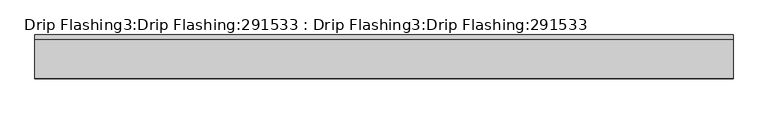
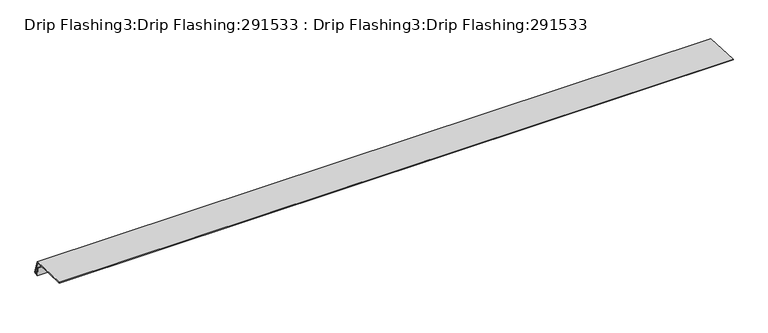
"""IFC4 building model written with IfcOpenShell, lengths in millimetres: proxy geometry, Drip Flashing3:Drip Flashing:291533 : Drip Flashing3:Drip Flashing:291533."""

from ifc_helpers import new_model, si_unit, frame, origin, place, context, project, spatial, polyline, outline, extrude, source, transform, mapped, element, save


def drip_flashing3_drip_flashing_291533_drip_flashing3_drip_993810a2(model_context):
    return source(origin(), model_context, "Body", "SweptSolid", [
        extrude(outline(polyline([(10061.8225481, 37565.8250877), (10050.7641618, 37602.7738382), (9938.445304, 37607.3484725), (9938.5314423, 37609.463386), (10052.3590143, 37604.8273034), (10064.452463, 37564.4201582), (10052.3732421, 37560.8049699), (10049.7522793, 37585.7417648), (10051.8407753, 37585.9612746), (10054.1970465, 37563.5428523), (10061.8225481, 37565.8250877)])), frame((-4455.0628198, 0.0, 0.0), z_axis=(1.0, 0.0, 0.0), x_axis=(0.0, 1.0, 0.0)), (0.0, 0.0, 1.0), 1999.85),
    ])


if __name__ == "__main__":
    model = new_model("IFC4")
    model_context = context("Model", 3, world=origin())
    ifc_project = project(units=[si_unit("LENGTHUNIT", "METRE", prefix="MILLI")], contexts=[model_context])
    site = spatial("IfcSite", under=ifc_project)
    building = spatial("IfcBuilding", under=site)
    placement = place(None, origin())
    drip_flashing3_drip_flashing_291533_drip_flashing3_drip_shape = drip_flashing3_drip_flashing_291533_drip_flashing3_drip_993810a2(model_context)
    element("IfcBuildingElementProxy", 1, Name="Drip Flashing3:Drip Flashing:291533 : Drip Flashing3:Drip Flashing:291533", ObjectType="Drip Flashing3:Drip Flashing:291533 : Drip Flashing3:Drip Flashing:291533", at=placement, inside=building, context=model_context, shape_type="MappedRepresentation", body=[
        mapped(drip_flashing3_drip_flashing_291533_drip_flashing3_drip_shape, transform((0.0, 0.0, 0.0), x_axis=(1.0, 0.0, 0.0), y_axis=(0.0, 1.0, 0.0), z_axis=(0.0, 0.0, 1.0))),
    ])
    save(model, "model.ifc")

# Revit data of these elements
# Type "Drip Flashing3:Drip Flashing:291533 : Drip Flashing3:Drip Flashing:291533"
#   NameOverride = "Drip Flashing3:Drip Flashing:291533"
#   ObjectTypeOverride = "Drip Flashing3:Drip Flashing"
#   Reference = "Drip Flashing"
#   Category = "Generic Models"
#   Tag = "291533"
# Element 1 (IfcBuildingElementProxy, "Drip Flashing3:Drip Flashing:291533 : Drip Flashing3:Drip Flashing:291533")
#   Materials on its faces: "DRIP FLASHING"
# Materials
#   "DRIP FLASHING": class "Unassigned", colour RGB 134 230 106, transparency 0, Cost = 0
